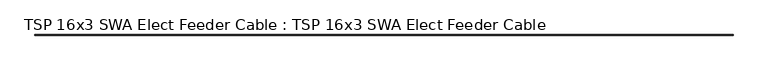
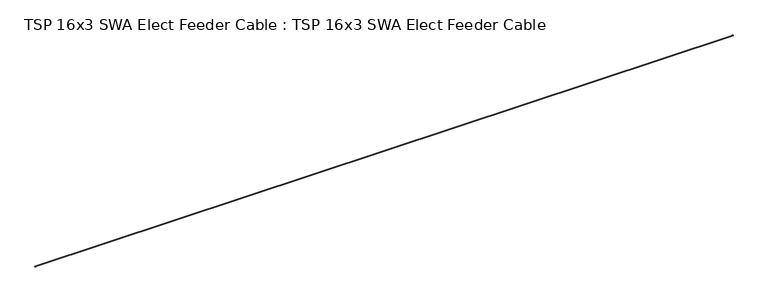
"""IFC4 building model written with IfcOpenShell, lengths in millimetres: proxy geometry, TSP 16x3 SWA Elect Feeder Cable : TSP 16x3 SWA Elect Feeder Cable."""

from ifc_helpers import new_model, si_unit, point, frame, frame_2d, origin, origin_2d, place, context, project, spatial, circle_curve, trimmed, segment, composite_curve, outline, extrude, source, transform, mapped, element, save


def tsp_16x3_swa_elect_feeder_cable_tsp_16x3_swa_elect_feeder_81bd3194(model_context):
    return source(origin(), model_context, "Body", "SweptSolid", [
        extrude(outline(composite_curve([segment(trimmed(circle_curve(origin_2d(), 30.0), [point((-30.0, 0.0))], [point((30.0, 0.0))], False, "CARTESIAN"), True, "CONTINUOUS"), segment(trimmed(circle_curve(origin_2d(), 30.0), [point((30.0, 0.0))], [point((-30.0, 0.0))], False, "CARTESIAN"), True, "CONTINUOUS")], self_intersect=False), holes=[composite_curve([segment(trimmed(circle_curve(origin_2d(), 27.0), [point((-27.0, 0.0))], [point((27.0, 0.0))], True, "CARTESIAN"), True, "CONTINUOUS"), segment(trimmed(circle_curve(origin_2d(), 27.0), [point((27.0, 0.0))], [point((-27.0, 0.0))], True, "CARTESIAN"), True, "CONTINUOUS")], self_intersect=False)]), frame((0.0, 0.0, 0.0), z_axis=(1.0, 0.0, 0.0), x_axis=(0.0, 1.0, 0.0)), (0.0, 0.0, 1.0), 66000.0),
        extrude(outline(composite_curve([segment(trimmed(circle_curve(frame_2d((11.691343, 6.75)), 8.0), [point((3.691343, 6.75))], [point((19.691343, 6.75))], False, "CARTESIAN"), True, "CONTINUOUS"), segment(trimmed(circle_curve(frame_2d((11.691343, 6.75)), 8.0), [point((19.691343, 6.75))], [point((3.691343, 6.75))], False, "CARTESIAN"), True, "CONTINUOUS")], self_intersect=False)), frame((0.0, 0.0, 0.0), z_axis=(1.0, 0.0, 0.0), x_axis=(0.0, 1.0, 0.0)), (0.0, 0.0, 1.0), 66000.0),
        extrude(outline(composite_curve([segment(trimmed(circle_curve(frame_2d((-11.691343, 6.75)), 8.0), [point((-19.691343, 6.75))], [point((-3.691343, 6.75))], False, "CARTESIAN"), True, "CONTINUOUS"), segment(trimmed(circle_curve(frame_2d((-11.691343, 6.75)), 8.0), [point((-3.691343, 6.75))], [point((-19.691343, 6.75))], False, "CARTESIAN"), True, "CONTINUOUS")], self_intersect=False)), frame((0.0, 0.0, 0.0), z_axis=(1.0, 0.0, 0.0), x_axis=(0.0, 1.0, 0.0)), (0.0, 0.0, 1.0), 66000.0),
        extrude(outline(composite_curve([segment(trimmed(circle_curve(frame_2d((0.0, -13.5)), 8.0), [point((-8.0, -13.5))], [point((8.0, -13.5))], False, "CARTESIAN"), True, "CONTINUOUS"), segment(trimmed(circle_curve(frame_2d((0.0, -13.5)), 8.0), [point((8.0, -13.5))], [point((-8.0, -13.5))], False, "CARTESIAN"), True, "CONTINUOUS")], self_intersect=False)), frame((0.0, 0.0, 0.0), z_axis=(1.0, 0.0, 0.0), x_axis=(0.0, 1.0, 0.0)), (0.0, 0.0, 1.0), 66000.0),
        extrude(outline(composite_curve([segment(trimmed(circle_curve(origin_2d(), 27.0), [point((27.0, 0.0))], [point((-27.0, 0.0))], False, "CARTESIAN"), True, "CONTINUOUS"), segment(trimmed(circle_curve(origin_2d(), 27.0), [point((-27.0, 0.0))], [point((27.0, 0.0))], False, "CARTESIAN"), True, "CONTINUOUS")], self_intersect=False), holes=[composite_curve([segment(trimmed(circle_curve(frame_2d((-11.691343, 6.75)), 8.0), [point((-3.691343, 6.75))], [point((-19.691343, 6.75))], True, "CARTESIAN"), True, "CONTINUOUS"), segment(trimmed(circle_curve(frame_2d((-11.691343, 6.75)), 8.0), [point((-19.691343, 6.75))], [point((-3.691343, 6.75))], True, "CARTESIAN"), True, "CONTINUOUS")], self_intersect=False), composite_curve([segment(trimmed(circle_curve(frame_2d((11.691343, 6.75)), 8.0), [point((3.691343, 6.75))], [point((19.691343, 6.75))], True, "CARTESIAN"), True, "CONTINUOUS"), segment(trimmed(circle_curve(frame_2d((11.691343, 6.75)), 8.0), [point((19.691343, 6.75))], [point((3.691343, 6.75))], True, "CARTESIAN"), True, "CONTINUOUS")], self_intersect=False), composite_curve([segment(trimmed(circle_curve(frame_2d((0.0, -13.5)), 8.0), [point((-8.0, -13.5))], [point((8.0, -13.5))], True, "CARTESIAN"), True, "CONTINUOUS"), segment(trimmed(circle_curve(frame_2d((0.0, -13.5)), 8.0), [point((8.0, -13.5))], [point((-8.0, -13.5))], True, "CARTESIAN"), True, "CONTINUOUS")], self_intersect=False)]), frame((0.0, 0.0, 0.0), z_axis=(1.0, 0.0, 0.0), x_axis=(0.0, 1.0, 0.0)), (0.0, 0.0, 1.0), 66000.0),
    ])


if __name__ == "__main__":
    model = new_model("IFC4")
    model_context = context("Model", 3, world=origin())
    ifc_project = project(units=[si_unit("LENGTHUNIT", "METRE", prefix="MILLI")], contexts=[model_context])
    site = spatial("IfcSite", under=ifc_project)
    building = spatial("IfcBuilding", under=site)
    placement = place(None, origin())
    tsp_16x3_swa_elect_feeder_cable_tsp_16x3_swa_elect_feeder_shape = tsp_16x3_swa_elect_feeder_cable_tsp_16x3_swa_elect_feeder_81bd3194(model_context)
    element("IfcBuildingElementProxy", 1, Name="TSP 16x3 SWA Elect Feeder Cable : TSP 16x3 SWA Elect Feeder Cable", ObjectType="TSP 16x3 SWA Elect Feeder Cable : TSP 16x3 SWA Elect Feeder Cable", at=placement, inside=building, context=model_context, shape_type="MappedRepresentation", body=[
        mapped(tsp_16x3_swa_elect_feeder_cable_tsp_16x3_swa_elect_feeder_shape, transform((0.0, 0.0, 0.0), x_axis=(1.0, 0.0, 0.0), y_axis=(0.0, 1.0, 0.0), z_axis=(0.0, 0.0, 1.0))),
    ])
    save(model, "model.ifc")

# Revit data of these elements
# Type "TSP 16x3 SWA Elect Feeder Cable : TSP 16x3 SWA Elect Feeder Cable"
#   Model = "TSP_ELECSC163"
#   built-in parameter 1001306 [instance default] = 3.93701 (stored number, unit not read)
#   Cable Length [instance default] = 1200 mm
#   Default Elevation = 0
# Element 1 (IfcBuildingElementProxy, "TSP 16x3 SWA Elect Feeder Cable : TSP 16x3 SWA Elect Feeder Cable")
#   built-in parameter 1001306 = 216.535 (stored number, unit not read)
#   Cable Length = 66000 mm
#   Materials on its faces: "Cellulose Fill", "Copper", "Laminate, Red, Matte"
# Materials
#   "Cellulose Fill": class "Generic", colour RGB 0 0 0, transparency 0, Description = "Cellulose loose fill", Cost = 0
#   "Copper": class "Metal", colour RGB 0 0 0, transparency 0, Description = "Copper, matte finish", Cost = 0
#   "Laminate, Red, Matte": class "Plastic", colour RGB 255 0 0, transparency 0, Description = "Plastic Laminate - Red, Matte", Cost = 0
